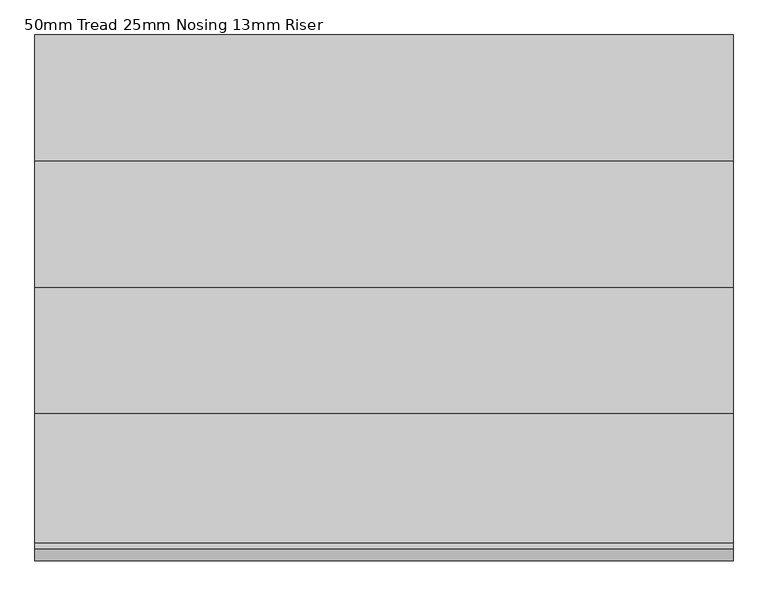
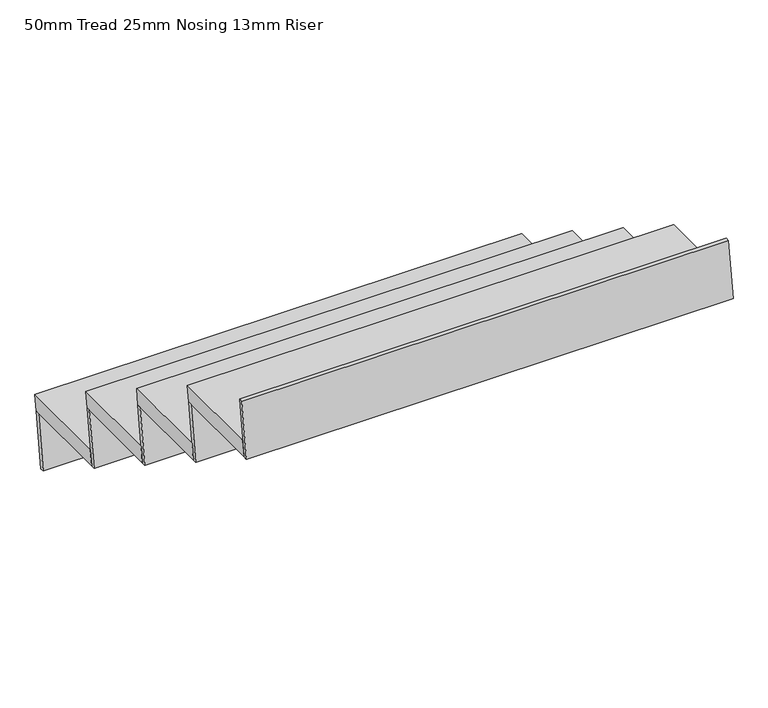
"""IFC4 building model written with IfcOpenShell, lengths in millimetres: stair flight geometry, 50mm Tread 25mm Nosing 13mm Riser."""

from ifc_helpers import new_model, si_unit, frame, origin, place, context, project, spatial, polyline, outline, extrude, source, transform, mapped, element, save


def stair_flight_50mm_tread_25mm_nosing_13mm_riser_f085b140(model_context):
    return source(origin(), model_context, "Body", "SweptSolid", [
        extrude(outline(polyline([(7032.4781803, 14794.1176471), (7332.4781803, 14794.1176471), (7325.3948469, 14744.1176471), (7025.3948469, 14744.1176471), (7032.4781803, 14794.1176471)])), frame((-226.7120949, 0.0, 0.0), z_axis=(1.0, 0.0, 0.0), x_axis=(0.0, 1.0, 0.0)), (0.0, 0.0, 1.0), 1520.0),
        extrude(outline(polyline([(7325.3948469, 14744.1176471), (7300.3948469, 14567.6470588), (7287.770036, 14567.6470588), (7312.770036, 14744.1176471), (7325.3948469, 14744.1176471)])), frame((-226.7120949, 0.0, 0.0), z_axis=(1.0, 0.0, 0.0), x_axis=(0.0, 1.0, 0.0)), (0.0, 0.0, 1.0), 1520.0),
        extrude(outline(polyline([(7050.3948469, 14920.5882353), (7025.3948469, 14744.1176471), (7012.770036, 14744.1176471), (7037.770036, 14920.5882353), (7050.3948469, 14920.5882353)])), frame((-226.7120949, 0.0, 0.0), z_axis=(1.0, 0.0, 0.0), x_axis=(0.0, 1.0, 0.0)), (0.0, 0.0, 1.0), 1520.0),
        extrude(outline(polyline([(6757.4781803, 14970.5882353), (7057.4781803, 14970.5882353), (7050.3948469, 14920.5882353), (6750.3948469, 14920.5882353), (6757.4781803, 14970.5882353)])), frame((-226.7120949, 0.0, 0.0), z_axis=(1.0, 0.0, 0.0), x_axis=(0.0, 1.0, 0.0)), (0.0, 0.0, 1.0), 1520.0),
        extrude(outline(polyline([(6775.3948469, 15097.0588235), (6750.3948469, 14920.5882353), (6737.770036, 14920.5882353), (6762.770036, 15097.0588235), (6775.3948469, 15097.0588235)])), frame((-226.7120949, 0.0, 0.0), z_axis=(1.0, 0.0, 0.0), x_axis=(0.0, 1.0, 0.0)), (0.0, 0.0, 1.0), 1520.0),
        extrude(outline(polyline([(6482.4781803, 15147.0588235), (6782.4781803, 15147.0588235), (6775.3948469, 15097.0588235), (6475.3948469, 15097.0588235), (6482.4781803, 15147.0588235)])), frame((-226.7120949, 0.0, 0.0), z_axis=(1.0, 0.0, 0.0), x_axis=(0.0, 1.0, 0.0)), (0.0, 0.0, 1.0), 1520.0),
        extrude(outline(polyline([(6500.3948469, 15273.5294118), (6475.3948469, 15097.0588235), (6462.770036, 15097.0588235), (6487.770036, 15273.5294118), (6500.3948469, 15273.5294118)])), frame((-226.7120949, 0.0, 0.0), z_axis=(1.0, 0.0, 0.0), x_axis=(0.0, 1.0, 0.0)), (0.0, 0.0, 1.0), 1520.0),
        extrude(outline(polyline([(6225.3948469, 15450.0), (6200.3948469, 15273.5294118), (6187.770036, 15273.5294118), (6212.770036, 15450.0), (6225.3948469, 15450.0)])), frame((-226.7120949, 0.0, 0.0), z_axis=(1.0, 0.0, 0.0), x_axis=(0.0, 1.0, 0.0)), (0.0, 0.0, 1.0), 1520.0),
        extrude(outline(polyline([(6207.4781803, 15323.5294118), (6507.4781803, 15323.5294118), (6500.3948469, 15273.5294118), (6200.3948469, 15273.5294118), (6207.4781803, 15323.5294118)])), frame((-226.7120949, 0.0, 0.0), z_axis=(1.0, 0.0, 0.0), x_axis=(0.0, 1.0, 0.0)), (0.0, 0.0, 1.0), 1520.0),
    ])


if __name__ == "__main__":
    model = new_model("IFC4")
    model_context = context("Model", 3, world=origin())
    ifc_project = project(units=[si_unit("LENGTHUNIT", "METRE", prefix="MILLI")], contexts=[model_context])
    site = spatial("IfcSite", under=ifc_project)
    building = spatial("IfcBuilding", under=site)
    placement = place(None, origin())
    stair_flight_50mm_tread_25mm_nosing_13mm_riser_shape = stair_flight_50mm_tread_25mm_nosing_13mm_riser_f085b140(model_context)
    element("IfcStairFlight", 1, ObjectType="50mm Tread 25mm Nosing 13mm Riser", at=placement, inside=building, context=model_context, shape_type="MappedRepresentation", body=[
        mapped(stair_flight_50mm_tread_25mm_nosing_13mm_riser_shape, transform((0.0, 0.0, 0.0), x_axis=(1.0, 0.0, 0.0), y_axis=(0.0, 1.0, 0.0), z_axis=(0.0, 0.0, 1.0))),
    ])
    save(model, "model.ifc")
